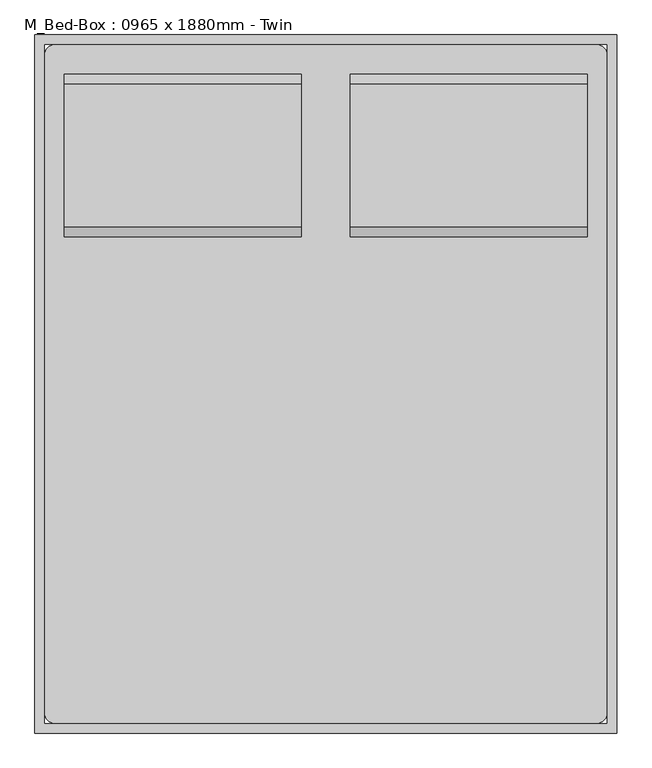
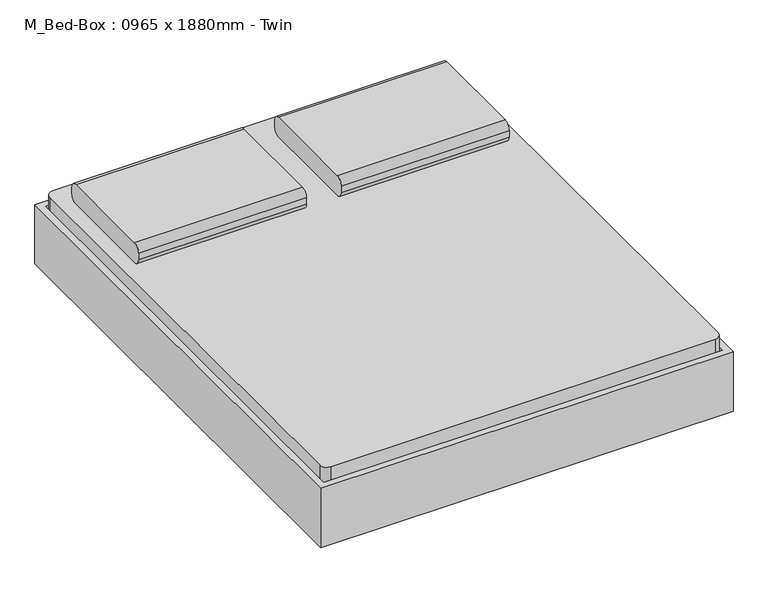
"""IFC4 building model written with IfcOpenShell, lengths in millimetres: furniture geometry, M_Bed-Box : 0965 x 1880mm - Twin."""

from ifc_helpers import new_model, si_unit, point, frame, frame_2d, origin, place, context, project, spatial, polyline, circle_curve, trimmed, segment, composite_curve, outline, extrude, source, transform, mapped, element, save
from ifc_brep_helpers import plane_surface, cylinder_surface, revolved_surface, advanced_brep


def m_bed_box_0965_x_1880mm_twin_f2e49195(model_context):
    return source(origin(), model_context, "Body", "SolidModel", [
        extrude(outline(composite_curve([segment(polyline([(538.5704918, 406.4), (170.2704918, 406.4)]), True, "CONTINUOUS"), segment(trimmed(circle_curve(frame_2d((170.2704918, 431.8)), 25.4), [point((170.2704918, 406.4))], [point((144.8704918, 431.8))], False, "CARTESIAN"), True, "CONTINUOUS"), segment(polyline([(144.8704918, 431.8), (144.8704918, 457.2)]), True, "CONTINUOUS"), segment(trimmed(circle_curve(frame_2d((170.2704918, 457.2)), 25.4), [point((144.8704918, 457.2))], [point((170.2704918, 482.6))], False, "CARTESIAN"), True, "CONTINUOUS"), segment(polyline([(170.2704918, 482.6), (538.5704918, 482.6)]), True, "CONTINUOUS"), segment(trimmed(circle_curve(frame_2d((538.5704918, 457.2)), 25.4), [point((538.5704918, 482.6))], [point((563.9704918, 457.2))], False, "CARTESIAN"), True, "CONTINUOUS"), segment(polyline([(563.9704918, 457.2), (563.9704918, 431.8)]), True, "CONTINUOUS"), segment(trimmed(circle_curve(frame_2d((538.5704918, 431.8)), 25.4), [point((563.9704918, 431.8))], [point((538.5704918, 406.4))], False, "CARTESIAN"), True, "CONTINUOUS")], self_intersect=False)), frame((402.652459, 0.0, 0.0), z_axis=(1.0, 0.0, 0.0), x_axis=(0.0, 1.0, 0.0)), (0.0, 0.0, 1.0), 610.3),
        extrude(outline(composite_curve([segment(polyline([(538.5704918, 406.4), (170.2704918, 406.4)]), True, "CONTINUOUS"), segment(trimmed(circle_curve(frame_2d((170.2704918, 431.8)), 25.4), [point((170.2704918, 406.4))], [point((144.8704918, 431.8))], False, "CARTESIAN"), True, "CONTINUOUS"), segment(polyline([(144.8704918, 431.8), (144.8704918, 457.2)]), True, "CONTINUOUS"), segment(trimmed(circle_curve(frame_2d((170.2704918, 457.2)), 25.4), [point((144.8704918, 457.2))], [point((170.2704918, 482.6))], False, "CARTESIAN"), True, "CONTINUOUS"), segment(polyline([(170.2704918, 482.6), (538.5704918, 482.6)]), True, "CONTINUOUS"), segment(trimmed(circle_curve(frame_2d((538.5704918, 457.2)), 25.4), [point((538.5704918, 482.6))], [point((563.9704918, 457.2))], False, "CARTESIAN"), True, "CONTINUOUS"), segment(polyline([(563.9704918, 457.2), (563.9704918, 431.8)]), True, "CONTINUOUS"), segment(trimmed(circle_curve(frame_2d((538.5704918, 431.8)), 25.4), [point((563.9704918, 431.8))], [point((538.5704918, 406.4))], False, "CARTESIAN"), True, "CONTINUOUS")], self_intersect=False)), frame((-334.647541, 0.0, 0.0), z_axis=(1.0, 0.0, 0.0), x_axis=(0.0, 1.0, 0.0)), (0.0, 0.0, 1.0), 610.3),
        advanced_brep(
        [(-385.1231784, 411.5704918, 177.8), (-385.1231784, 335.3704918, 177.8), (-385.1231784, 335.3704918, 196.85), (-385.1231784, 411.5704918, 196.85), (-334.3231784, 411.5704918, 177.8), (-334.3231784, 335.3704918, 177.8), (-322.1869899, 335.3704918, 196.85), (-322.1869899, 411.5704918, 196.85), (-258.2523099, 411.5704918, 14.6654962), (-258.2523099, 335.3704918, 14.6654962), (-240.9871466, 335.3704918, 22.716374), (-240.9871466, 411.5704918, 22.716374), (-235.2320921, 335.3704918, 0.0), (-235.2320921, 411.5704918, 0.0), (-235.2320921, 335.3704918, 19.05), (-235.2320921, 411.5704918, 19.05), (-156.6195862, 411.5704918, 0.0), (-156.6195862, 335.3704918, 0.0), (-156.6195862, 335.3704918, 19.05), (-156.6195862, 411.5704918, 19.05), (-143.9195862, 335.3704918, 3.4029547), (-143.9195862, 411.5704918, 3.4029547), (-153.4445862, 335.3704918, 19.9007387), (-153.4445862, 411.5704918, 19.9007387), (-83.822541, 411.5704918, 38.1), (-83.822541, 335.3704918, 38.1), (-88.9269731, 335.3704918, 57.15), (-88.9269731, 411.5704918, 57.15), (762.4518216, 411.5704918, 38.1), (762.4518216, 335.3704918, 38.1), (767.5562537, 335.3704918, 57.15), (767.5562537, 411.5704918, 57.15), (822.5488669, 411.5704918, 3.4029547), (822.5488669, 335.3704918, 3.4029547), (832.0738669, 335.3704918, 19.9007387), (832.0738669, 411.5704918, 19.9007387), (835.2488669, 335.3704918, 0.0), (835.2488669, 411.5704918, 0.0), (835.2488669, 335.3704918, 19.05), (835.2488669, 411.5704918, 19.05), (913.8613728, 411.5704918, 0.0), (913.8613728, 335.3704918, 0.0), (913.8613728, 335.3704918, 19.05), (913.8613728, 411.5704918, 19.05), (936.8815906, 335.3704918, 14.6654962), (936.8815906, 411.5704918, 14.6654962), (919.6164272, 335.3704918, 22.716374), (919.6164272, 411.5704918, 22.716374), (1012.952459, 411.5704918, 177.8), (1012.952459, 335.3704918, 177.8), (1000.8162705, 335.3704918, 196.85), (1000.8162705, 411.5704918, 196.85), (1063.752459, 411.5704918, 177.8), (1063.752459, 411.5704918, 196.85), (1063.752459, 335.3704918, 196.85), (1063.752459, 335.3704918, 177.8)],
        [
            (0, 1),
            (1, 2),
            (2, 3),
            (3, 0),
            (0, 4),
            (4, 5),
            (5, 1),
            (5, 6),
            (6, 2),
            (6, 7),
            (7, 3),
            (7, 4),
            (4, 8),
            (8, 9),
            (9, 5),
            (9, 10),
            (10, 6),
            (10, 11),
            (11, 7),
            (11, 8),
            (12, 9, circle_curve(frame((-235.2320921, 335.3704918, 25.4), z_axis=(0.0, 1.0, 0.0), x_axis=(-0.9063077870366488, 0.0, -0.4226182617407019)), 25.4)),
            (8, 13, circle_curve(frame((-235.2320921, 411.5704918, 25.4), z_axis=(0.0, -1.0, 0.0), x_axis=(-0.9063077870366488, 0.0, -0.4226182617407019)), 25.4)),
            (13, 12),
            (14, 10, circle_curve(frame((-235.2320921, 335.3704918, 25.4), z_axis=(0.0, 1.0, 0.0), x_axis=(-0.9063077870366488, 0.0, -0.4226182617407019)), 6.35)),
            (12, 14),
            (15, 11, circle_curve(frame((-235.2320921, 411.5704918, 25.4), z_axis=(0.0, 1.0, 0.0), x_axis=(-0.9063077870366488, 0.0, -0.4226182617407019)), 6.35)),
            (14, 15),
            (15, 13),
            (13, 16),
            (16, 17),
            (17, 12),
            (17, 18),
            (18, 14),
            (18, 19),
            (19, 15),
            (19, 16),
            (20, 17, circle_curve(frame((-156.6195862, 335.3704918, 25.4), z_axis=(0.0, 1.0, 0.0), x_axis=(0.0, 0.0, -1.0)), 25.4)),
            (16, 21, circle_curve(frame((-156.6195862, 411.5704918, 25.4), z_axis=(0.0, -1.0, 0.0), x_axis=(0.0, 0.0, -1.0)), 25.4)),
            (21, 20),
            (22, 18, circle_curve(frame((-156.6195862, 335.3704918, 25.4), z_axis=(0.0, 1.0, 0.0), x_axis=(0.0, 0.0, -1.0)), 6.35)),
            (20, 22),
            (23, 19, circle_curve(frame((-156.6195862, 411.5704918, 25.4), z_axis=(0.0, 1.0, 0.0), x_axis=(0.0, 0.0, -1.0)), 6.35)),
            (22, 23),
            (23, 21),
            (21, 24),
            (24, 25),
            (25, 20),
            (25, 26),
            (26, 22),
            (26, 27),
            (27, 23),
            (27, 24),
            (24, 28),
            (28, 29),
            (29, 25),
            (29, 30),
            (30, 26),
            (30, 31),
            (31, 27),
            (31, 28),
            (28, 32),
            (32, 33),
            (33, 29),
            (33, 34),
            (34, 30),
            (34, 35),
            (35, 31),
            (35, 32),
            (36, 33, circle_curve(frame((835.2488669, 335.3704918, 25.4), z_axis=(0.0, 1.0, 0.0), x_axis=(-0.5000000000000463, 0.0, -0.8660254037844118)), 25.4)),
            (32, 37, circle_curve(frame((835.2488669, 411.5704918, 25.4), z_axis=(0.0, -1.0, 0.0), x_axis=(-0.5000000000000463, 0.0, -0.8660254037844118)), 25.4)),
            (37, 36),
            (38, 34, circle_curve(frame((835.2488669, 335.3704918, 25.4), z_axis=(0.0, 1.0, 0.0), x_axis=(-0.5000000000000463, 0.0, -0.8660254037844118)), 6.35)),
            (36, 38),
            (39, 35, circle_curve(frame((835.2488669, 411.5704918, 25.4), z_axis=(0.0, 1.0, 0.0), x_axis=(-0.5000000000000463, 0.0, -0.8660254037844118)), 6.35)),
            (38, 39),
            (39, 37),
            (37, 40),
            (40, 41),
            (41, 36),
            (41, 42),
            (42, 38),
            (42, 43),
            (43, 39),
            (43, 40),
            (44, 41, circle_curve(frame((913.8613728, 335.3704918, 25.4), z_axis=(0.0, 1.0, 0.0), x_axis=(0.0, 0.0, -1.0)), 25.4)),
            (40, 45, circle_curve(frame((913.8613728, 411.5704918, 25.4), z_axis=(0.0, -1.0, 0.0), x_axis=(0.0, 0.0, -1.0)), 25.4)),
            (45, 44),
            (46, 42, circle_curve(frame((913.8613728, 335.3704918, 25.4), z_axis=(0.0, 1.0, 0.0), x_axis=(0.0, 0.0, -1.0)), 6.35)),
            (44, 46),
            (47, 43, circle_curve(frame((913.8613728, 411.5704918, 25.4), z_axis=(0.0, 1.0, 0.0), x_axis=(0.0, 0.0, -1.0)), 6.35)),
            (46, 47),
            (47, 45),
            (45, 48),
            (48, 49),
            (49, 44),
            (49, 50),
            (50, 46),
            (50, 51),
            (51, 47),
            (51, 48),
            (52, 53),
            (53, 54),
            (54, 55),
            (55, 52),
            (48, 52),
            (55, 49),
            (54, 50),
            (53, 51),
        ],
        [
            plane_surface(frame((-385.1231784, 665.5704918, -152.9490627), z_axis=(-1.0, 0.0, 0.0), x_axis=(0.0, 1.0, 0.0))),
            plane_surface(frame((-385.1231784, 411.5704918, 177.8), z_axis=(0.0, 0.0, -1.0), x_axis=(1.0, 0.0, 0.0))),
            plane_surface(frame((-385.1231784, 335.3704918, 177.8), z_axis=(0.0, -1.0, 0.0), x_axis=(1.0, 0.0, 0.0))),
            plane_surface(frame((-385.1231784, 335.3704918, 196.85), z_axis=(0.0, 0.0, 1.0), x_axis=(1.0, 0.0, 0.0))),
            plane_surface(frame((-385.1231784, 411.5704918, 196.85), z_axis=(0.0, 1.0, 0.0), x_axis=(1.0, 0.0, 0.0))),
            plane_surface(frame((-334.3231784, 411.5704918, 177.8), z_axis=(-0.9063077870366485, 0.0, -0.4226182617407027), x_axis=(0.4226182617407027, 0.0, -0.9063077870366485))),
            plane_surface(frame((-334.3231784, 335.3704918, 177.8), z_axis=(0.0, -1.0, 0.0), x_axis=(0.4226182617407027, 0.0, -0.9063077870366485))),
            plane_surface(frame((-322.1869899, 335.3704918, 196.85), z_axis=(0.9063077870366486, 0.0, 0.4226182617407026), x_axis=(0.4226182617407026, 0.0, -0.9063077870366486))),
            plane_surface(frame((-322.1869899, 411.5704918, 196.85), z_axis=(0.0, 1.0, 0.0), x_axis=(0.4226182617407027, 0.0, -0.9063077870366485))),
            cylinder_surface(frame((-235.2320921, 665.5704918, 25.4), z_axis=(0.0, -1.0, 0.0), x_axis=(-0.9063077870366488, 0.0, -0.4226182617407019)), 25.4),
            plane_surface(frame((-235.2320921, 335.3704918, 25.4), z_axis=(0.0, -1.0, 0.0), x_axis=(-0.9063077870366488, 0.0, -0.4226182617407019))),
            revolved_surface(polyline([(-240.9871465476827, 335.3704918, 22.716374037946544), (-240.9871465476827, 411.5704918, 22.716374037946544)]), (-235.2320921, 665.5704918, 25.4), (0.0, -1.0, 0.0)),
            plane_surface(frame((-235.2320921, 411.5704918, 25.4), z_axis=(0.0, 1.0, 0.0), x_axis=(-0.9063077870366488, 0.0, -0.4226182617407019))),
            plane_surface(frame((-235.2320921, 411.5704918, 0.0), z_axis=(0.0, 0.0, -1.0), x_axis=(1.0, 0.0, 0.0))),
            plane_surface(frame((-235.2320921, 335.3704918, 0.0), z_axis=(0.0, -1.0, 0.0), x_axis=(1.0, 0.0, 0.0))),
            plane_surface(frame((-235.2320921, 335.3704918, 19.05), z_axis=(0.0, 0.0, 1.0), x_axis=(1.0, 0.0, 0.0))),
            plane_surface(frame((-235.2320921, 411.5704918, 19.05), z_axis=(0.0, 1.0, 0.0), x_axis=(1.0, 0.0, 0.0))),
            cylinder_surface(frame((-156.6195862, 665.5704918, 25.4), z_axis=(0.0, -1.0, 0.0), x_axis=(0.0, 0.0, -1.0)), 25.4),
            plane_surface(frame((-156.6195862, 335.3704918, 25.4), z_axis=(0.0, -1.0, 0.0), x_axis=(0.0, 0.0, -1.0))),
            revolved_surface(polyline([(-156.6195862, 335.3704918, 19.049999999999997), (-156.6195862, 411.5704918, 19.049999999999997)]), (-156.6195862, 665.5704918, 25.4), (0.0, -1.0, 0.0)),
            plane_surface(frame((-156.6195862, 411.5704918, 25.4), z_axis=(0.0, 1.0, 0.0), x_axis=(0.0, 0.0, -1.0))),
            plane_surface(frame((-143.9195862, 411.5704918, 3.4029547), z_axis=(0.4999999999998775, 0.0, -0.8660254037845093), x_axis=(0.8660254037845093, 0.0, 0.4999999999998775))),
            plane_surface(frame((-143.9195862, 335.3704918, 3.4029547), z_axis=(0.0, -1.0, 0.0), x_axis=(0.8660254037845092, 0.0, 0.49999999999987776))),
            plane_surface(frame((-153.4445862, 335.3704918, 19.9007387), z_axis=(-0.4999999999998776, 0.0, 0.8660254037845093), x_axis=(0.8660254037845093, 0.0, 0.4999999999998776))),
            plane_surface(frame((-153.4445862, 411.5704918, 19.9007387), z_axis=(0.0, 1.0, 0.0), x_axis=(0.8660254037845095, 0.0, 0.4999999999998772))),
            plane_surface(frame((-83.822541, 411.5704918, 38.1), z_axis=(0.0, 0.0, -1.0), x_axis=(1.0, 0.0, 0.0))),
            plane_surface(frame((-83.822541, 335.3704918, 38.1), z_axis=(0.0, -1.0, 0.0), x_axis=(1.0, 0.0, 0.0))),
            plane_surface(frame((-88.9269731, 335.3704918, 57.15), z_axis=(0.0, 0.0, 1.0), x_axis=(1.0, 0.0, 0.0))),
            plane_surface(frame((-88.9269731, 411.5704918, 57.15), z_axis=(0.0, 1.0, 0.0), x_axis=(1.0, 0.0, 0.0))),
            plane_surface(frame((762.4518216, 411.5704918, 38.1), z_axis=(-0.5000000000000455, 0.0, -0.8660254037844124), x_axis=(0.8660254037844124, 0.0, -0.5000000000000455))),
            plane_surface(frame((762.4518216, 335.3704918, 38.1), z_axis=(0.0, -1.0000000000000002, 0.0), x_axis=(0.8660254037844132, 0.0, -0.5000000000000443))),
            plane_surface(frame((767.5562537, 335.3704918, 57.15), z_axis=(0.500000000000045, 0.0, 0.8660254037844127), x_axis=(0.8660254037844127, 0.0, -0.500000000000045))),
            plane_surface(frame((767.5562537, 411.5704918, 57.15), z_axis=(0.0, 1.0000000000000002, 0.0), x_axis=(0.8660254037844123, 0.0, -0.5000000000000459))),
            cylinder_surface(frame((835.2488669, 665.5704918, 25.4), z_axis=(0.0, -1.0, 0.0), x_axis=(-0.5000000000000463, 0.0, -0.8660254037844118)), 25.4),
            plane_surface(frame((835.2488669, 335.3704918, 25.4), z_axis=(0.0, -1.0000000000000002, 0.0), x_axis=(-0.5000000000000464, 0.0, -0.866025403784412))),
            revolved_surface(polyline([(832.0738668999998, 335.3704918, 19.90073868596898), (832.0738668999998, 411.5704918, 19.90073868596898)]), (835.2488669, 665.5704918, 25.4), (0.0, -1.0, 0.0)),
            plane_surface(frame((835.2488669, 411.5704918, 25.4), z_axis=(0.0, 1.0000000000000002, 0.0), x_axis=(-0.5000000000000464, 0.0, -0.866025403784412))),
            plane_surface(frame((835.2488669, 411.5704918, 0.0), z_axis=(0.0, 0.0, -1.0), x_axis=(1.0, 0.0, 0.0))),
            plane_surface(frame((835.2488669, 335.3704918, 0.0), z_axis=(0.0, -1.0, 0.0), x_axis=(1.0, 0.0, 0.0))),
            plane_surface(frame((835.2488669, 335.3704918, 19.05), z_axis=(0.0, 0.0, 1.0), x_axis=(1.0, 0.0, 0.0))),
            plane_surface(frame((835.2488669, 411.5704918, 19.05), z_axis=(0.0, 1.0, 0.0), x_axis=(1.0, 0.0, 0.0))),
            cylinder_surface(frame((913.8613728, 665.5704918, 25.4), z_axis=(0.0, -1.0, 0.0), x_axis=(0.0, 0.0, -1.0)), 25.4),
            plane_surface(frame((913.8613728, 335.3704918, 25.4), z_axis=(0.0, -1.0, 0.0), x_axis=(0.0, 0.0, -1.0))),
            revolved_surface(polyline([(913.8613728, 335.3704918, 19.049999999999997), (913.8613728, 411.5704918, 19.049999999999997)]), (913.8613728, 665.5704918, 25.4), (0.0, -1.0, 0.0)),
            plane_surface(frame((913.8613728, 411.5704918, 25.4), z_axis=(0.0, 1.0, 0.0), x_axis=(0.0, 0.0, -1.0))),
            plane_surface(frame((936.8815906, 411.5704918, 14.6654962), z_axis=(0.9063077870366809, 0.0, -0.42261826174063305), x_axis=(0.42261826174063305, 0.0, 0.9063077870366809))),
            plane_surface(frame((936.8815906, 335.3704918, 14.6654962), z_axis=(0.0, -1.0, 0.0), x_axis=(0.4226182617406331, 0.0, 0.9063077870366809))),
            plane_surface(frame((919.6164272, 335.3704918, 22.716374), z_axis=(-0.9063077870366807, 0.0, 0.4226182617406336), x_axis=(0.4226182617406336, 0.0, 0.9063077870366807))),
            plane_surface(frame((919.6164272, 411.5704918, 22.716374), z_axis=(0.0, 1.0000000000000002, 0.0), x_axis=(0.422618261740634, 0.0, 0.9063077870366806))),
            plane_surface(frame((1063.752459, 665.5704918, -152.9490627), z_axis=(1.0, 0.0, 0.0), x_axis=(0.0, 1.0, 0.0))),
            plane_surface(frame((1012.952459, 411.5704918, 177.8), z_axis=(0.0, 0.0, -1.0), x_axis=(1.0, 0.0, 0.0))),
            plane_surface(frame((1012.952459, 335.3704918, 177.8), z_axis=(0.0, -1.0, 0.0), x_axis=(1.0, 0.0, 0.0))),
            plane_surface(frame((1000.8162705, 335.3704918, 196.85), z_axis=(0.0, 0.0, 1.0), x_axis=(1.0, 0.0, 0.0))),
            plane_surface(frame((1000.8162705, 411.5704918, 196.85), z_axis=(0.0, 1.0, 0.0), x_axis=(1.0, 0.0, 0.0))),
        ],
        [
            (0, [[1, 2, 3, 4]]),
            (1, [[-1, 5, 6, 7]]),
            (2, [[-2, -7, 8, 9]]),
            (3, [[-3, -9, 10, 11]]),
            (4, [[-4, -11, 12, -5]]),
            (5, [[-6, 13, 14, 15]]),
            (6, [[-8, -15, 16, 17]]),
            (7, [[-10, -17, 18, 19]]),
            (8, [[-12, -19, 20, -13]]),
            (9, [[21, -14, 22, 23]]),
            (10, [[24, -16, -21, 25]]),
            (11, [[26, -18, -24, 27]]),
            (12, [[-22, -20, -26, 28]]),
            (13, [[-23, 29, 30, 31]]),
            (14, [[-25, -31, 32, 33]]),
            (15, [[-27, -33, 34, 35]]),
            (16, [[-28, -35, 36, -29]]),
            (17, [[37, -30, 38, 39]]),
            (18, [[40, -32, -37, 41]]),
            (19, [[42, -34, -40, 43]]),
            (20, [[-38, -36, -42, 44]]),
            (21, [[-39, 45, 46, 47]]),
            (22, [[-41, -47, 48, 49]]),
            (23, [[-43, -49, 50, 51]]),
            (24, [[-44, -51, 52, -45]]),
            (25, [[-46, 53, 54, 55]]),
            (26, [[-48, -55, 56, 57]]),
            (27, [[-50, -57, 58, 59]]),
            (28, [[-52, -59, 60, -53]]),
            (29, [[-54, 61, 62, 63]]),
            (30, [[-56, -63, 64, 65]]),
            (31, [[-58, -65, 66, 67]]),
            (32, [[-60, -67, 68, -61]]),
            (33, [[69, -62, 70, 71]]),
            (34, [[72, -64, -69, 73]]),
            (35, [[74, -66, -72, 75]]),
            (36, [[-70, -68, -74, 76]]),
            (37, [[-71, 77, 78, 79]]),
            (38, [[-73, -79, 80, 81]]),
            (39, [[-75, -81, 82, 83]]),
            (40, [[-76, -83, 84, -77]]),
            (41, [[85, -78, 86, 87]]),
            (42, [[88, -80, -85, 89]]),
            (43, [[90, -82, -88, 91]]),
            (44, [[-86, -84, -90, 92]]),
            (45, [[-87, 93, 94, 95]]),
            (46, [[-89, -95, 96, 97]]),
            (47, [[-91, -97, 98, 99]]),
            (48, [[-92, -99, 100, -93]]),
            (49, [[101, 102, 103, 104]]),
            (50, [[-94, 105, -104, 106]]),
            (51, [[-96, -106, -103, 107]]),
            (52, [[-98, -107, -102, 108]]),
            (53, [[-100, -108, -101, -105]]),
        ],
    ),
        extrude(outline(composite_curve([segment(polyline([(-360.047541, 640.1704918), (1038.352459, 640.1704918)]), True, "CONTINUOUS"), segment(trimmed(circle_curve(frame_2d((1038.352459, 614.7704918)), 25.4), [point((1038.352459, 640.1704918))], [point((1063.752459, 614.7704918))], False, "CARTESIAN"), True, "CONTINUOUS"), segment(polyline([(1063.752459, 614.7704918), (1063.752459, -1083.6295082)]), True, "CONTINUOUS"), segment(trimmed(circle_curve(frame_2d((1038.352459, -1083.6295082)), 25.4), [point((1063.752459, -1083.6295082))], [point((1038.352459, -1109.0295082))], False, "CARTESIAN"), True, "CONTINUOUS"), segment(polyline([(1038.352459, -1109.0295082), (-360.047541, -1109.0295082)]), True, "CONTINUOUS"), segment(trimmed(circle_curve(frame_2d((-360.047541, -1083.6295082)), 25.4), [point((-360.047541, -1109.0295082))], [point((-385.447541, -1083.6295082))], False, "CARTESIAN"), True, "CONTINUOUS"), segment(polyline([(-385.447541, -1083.6295082), (-385.447541, 614.7704918)]), True, "CONTINUOUS"), segment(trimmed(circle_curve(frame_2d((-360.047541, 614.7704918)), 25.4), [point((-385.447541, 614.7704918))], [point((-360.047541, 640.1704918))], False, "CARTESIAN"), True, "CONTINUOUS")], self_intersect=False)), frame((0.0, 0.0, 203.2), z_axis=(0.0, 0.0, 1.0), x_axis=(1.0, 0.0, 0.0)), (0.0, 0.0, 1.0), 203.2),
        advanced_brep(
        [(-385.447541, -829.6295082, 196.85), (-385.447541, -829.6295082, 177.8), (-385.447541, -905.8295082, 177.8), (-385.447541, -905.8295082, 196.85), (-322.5113525, -829.6295082, 196.85), (-334.647541, -829.6295082, 177.8), (-334.647541, -905.8295082, 177.8), (-322.5113525, -905.8295082, 196.85), (-241.3115092, -829.6295082, 22.716374), (-258.5766725, -829.6295082, 14.6654962), (-258.5766725, -905.8295082, 14.6654962), (-241.3115092, -905.8295082, 22.716374), (-235.5564547, -829.6295082, 0.0), (-235.5564547, -829.6295082, 19.05), (-235.5564547, -905.8295082, 0.0), (-235.5564547, -905.8295082, 19.05), (-156.9439489, -829.6295082, 19.05), (-156.9439489, -829.6295082, 0.0), (-156.9439489, -905.8295082, 0.0), (-156.9439489, -905.8295082, 19.05), (-144.2439489, -829.6295082, 3.4029547), (-153.7689489, -829.6295082, 19.9007387), (-144.2439489, -905.8295082, 3.4029547), (-153.7689489, -905.8295082, 19.9007387), (-89.2513357, -829.6295082, 57.15), (-84.1469036, -829.6295082, 38.1), (-84.1469036, -905.8295082, 38.1), (-89.2513357, -905.8295082, 57.15), (767.5562537, -829.6295082, 57.15), (762.4518216, -829.6295082, 38.1), (762.4518216, -905.8295082, 38.1), (767.5562537, -905.8295082, 57.15), (832.0738669, -829.6295082, 19.9007387), (822.5488669, -829.6295082, 3.4029547), (822.5488669, -905.8295082, 3.4029547), (832.0738669, -905.8295082, 19.9007387), (835.2488669, -829.6295082, 0.0), (835.2488669, -829.6295082, 19.05), (835.2488669, -905.8295082, 0.0), (835.2488669, -905.8295082, 19.05), (913.8613728, -829.6295082, 19.05), (913.8613728, -829.6295082, 0.0), (913.8613728, -905.8295082, 0.0), (913.8613728, -905.8295082, 19.05), (936.8815906, -829.6295082, 14.6654962), (919.6164272, -829.6295082, 22.716374), (936.8815906, -905.8295082, 14.6654962), (919.6164272, -905.8295082, 22.716374), (1000.8162705, -829.6295082, 196.85), (1012.952459, -829.6295082, 177.8), (1012.952459, -905.8295082, 177.8), (1000.8162705, -905.8295082, 196.85), (1063.752459, -829.6295082, 196.85), (1063.752459, -905.8295082, 196.85), (1063.752459, -905.8295082, 177.8), (1063.752459, -829.6295082, 177.8)],
        [
            (0, 1),
            (1, 2),
            (2, 3),
            (3, 0),
            (0, 4),
            (4, 5),
            (5, 1),
            (5, 6),
            (6, 2),
            (6, 7),
            (7, 3),
            (7, 4),
            (4, 8),
            (8, 9),
            (9, 5),
            (9, 10),
            (10, 6),
            (10, 11),
            (11, 7),
            (11, 8),
            (12, 9, circle_curve(frame((-235.5564547, -829.6295082, 25.4), z_axis=(0.0, 1.0, 0.0), x_axis=(-0.906307787036664, 0.0, -0.4226182617406693)), 25.4)),
            (8, 13, circle_curve(frame((-235.5564547, -829.6295082, 25.4), z_axis=(0.0, -1.0, 0.0), x_axis=(-0.906307787036664, 0.0, -0.4226182617406693)), 6.35)),
            (13, 12),
            (14, 10, circle_curve(frame((-235.5564547, -905.8295082, 25.4), z_axis=(0.0, 1.0, 0.0), x_axis=(-0.906307787036664, 0.0, -0.4226182617406693)), 25.4)),
            (12, 14),
            (15, 11, circle_curve(frame((-235.5564547, -905.8295082, 25.4), z_axis=(0.0, 1.0, 0.0), x_axis=(-0.906307787036664, 0.0, -0.4226182617406693)), 6.35)),
            (14, 15),
            (15, 13),
            (13, 16),
            (16, 17),
            (17, 12),
            (17, 18),
            (18, 14),
            (18, 19),
            (19, 15),
            (19, 16),
            (20, 17, circle_curve(frame((-156.9439489, -829.6295082, 25.4), z_axis=(0.0, 1.0, 0.0), x_axis=(0.0, 0.0, -1.0)), 25.4)),
            (16, 21, circle_curve(frame((-156.9439489, -829.6295082, 25.4), z_axis=(0.0, -1.0, 0.0), x_axis=(0.0, 0.0, -1.0)), 6.35)),
            (21, 20),
            (22, 18, circle_curve(frame((-156.9439489, -905.8295082, 25.4), z_axis=(0.0, 1.0, 0.0), x_axis=(0.0, 0.0, -1.0)), 25.4)),
            (20, 22),
            (23, 19, circle_curve(frame((-156.9439489, -905.8295082, 25.4), z_axis=(0.0, 1.0, 0.0), x_axis=(0.0, 0.0, -1.0)), 6.35)),
            (22, 23),
            (23, 21),
            (21, 24),
            (24, 25),
            (25, 20),
            (25, 26),
            (26, 22),
            (26, 27),
            (27, 23),
            (27, 24),
            (24, 28),
            (28, 29),
            (29, 25),
            (29, 30),
            (30, 26),
            (30, 31),
            (31, 27),
            (31, 28),
            (28, 32),
            (32, 33),
            (33, 29),
            (33, 34),
            (34, 30),
            (34, 35),
            (35, 31),
            (35, 32),
            (36, 33, circle_curve(frame((835.2488669, -829.6295082, 25.4), z_axis=(0.0, 1.0, 0.0), x_axis=(-0.5000000000000525, 0.0, -0.8660254037844083)), 25.4)),
            (32, 37, circle_curve(frame((835.2488669, -829.6295082, 25.4), z_axis=(0.0, -1.0, 0.0), x_axis=(-0.5000000000000525, 0.0, -0.8660254037844083)), 6.35)),
            (37, 36),
            (38, 34, circle_curve(frame((835.2488669, -905.8295082, 25.4), z_axis=(0.0, 1.0, 0.0), x_axis=(-0.5000000000000525, 0.0, -0.8660254037844083)), 25.4)),
            (36, 38),
            (39, 35, circle_curve(frame((835.2488669, -905.8295082, 25.4), z_axis=(0.0, 1.0, 0.0), x_axis=(-0.5000000000000525, 0.0, -0.8660254037844083)), 6.35)),
            (38, 39),
            (39, 37),
            (37, 40),
            (40, 41),
            (41, 36),
            (41, 42),
            (42, 38),
            (42, 43),
            (43, 39),
            (43, 40),
            (44, 41, circle_curve(frame((913.8613728, -829.6295082, 25.4), z_axis=(0.0, 1.0, 0.0), x_axis=(0.0, 0.0, -1.0)), 25.4)),
            (40, 45, circle_curve(frame((913.8613728, -829.6295082, 25.4), z_axis=(0.0, -1.0, 0.0), x_axis=(0.0, 0.0, -1.0)), 6.35)),
            (45, 44),
            (46, 42, circle_curve(frame((913.8613728, -905.8295082, 25.4), z_axis=(0.0, 1.0, 0.0), x_axis=(0.0, 0.0, -1.0)), 25.4)),
            (44, 46),
            (47, 43, circle_curve(frame((913.8613728, -905.8295082, 25.4), z_axis=(0.0, 1.0, 0.0), x_axis=(0.0, 0.0, -1.0)), 6.35)),
            (46, 47),
            (47, 45),
            (45, 48),
            (48, 49),
            (49, 44),
            (49, 50),
            (50, 46),
            (50, 51),
            (51, 47),
            (51, 48),
            (52, 53),
            (53, 54),
            (54, 55),
            (55, 52),
            (48, 52),
            (55, 49),
            (54, 50),
            (53, 51),
        ],
        [
            plane_surface(frame((-385.447541, -1134.4295082, -127.5947323), z_axis=(-1.0, 0.0, 0.0), x_axis=(0.0, 1.0, 0.0))),
            plane_surface(frame((-385.447541, -829.6295082, 196.85), z_axis=(0.0, 1.0, 0.0), x_axis=(1.0, 0.0, 0.0))),
            plane_surface(frame((-385.447541, -829.6295082, 177.8), z_axis=(0.0, 0.0, -1.0), x_axis=(1.0, 0.0, 0.0))),
            plane_surface(frame((-385.447541, -905.8295082, 177.8), z_axis=(0.0, -1.0, 0.0), x_axis=(1.0, 0.0, 0.0))),
            plane_surface(frame((-385.447541, -905.8295082, 196.85), z_axis=(0.0, 0.0, 1.0), x_axis=(1.0, 0.0, 0.0))),
            plane_surface(frame((-322.5113525, -829.6295082, 196.85), z_axis=(0.0, 1.0000000000000002, 0.0), x_axis=(0.42261826174067135, 0.0, -0.9063077870366631))),
            plane_surface(frame((-334.647541, -829.6295082, 177.8), z_axis=(-0.906307787036663, 0.0, -0.42261826174067146), x_axis=(0.42261826174067146, 0.0, -0.906307787036663))),
            plane_surface(frame((-334.647541, -905.8295082, 177.8), z_axis=(0.0, -1.0, 0.0), x_axis=(0.42261826174067174, 0.0, -0.9063077870366629))),
            plane_surface(frame((-322.5113525, -905.8295082, 196.85), z_axis=(0.906307787036663, 0.0, 0.4226182617406716), x_axis=(0.4226182617406716, 0.0, -0.906307787036663))),
            plane_surface(frame((-235.5564547, -829.6295082, 25.4), z_axis=(0.0, 1.0, 0.0), x_axis=(-0.906307787036664, 0.0, -0.4226182617406693))),
            cylinder_surface(frame((-235.5564547, -1134.4295082, 25.4), z_axis=(0.0, -1.0, 0.0), x_axis=(-0.906307787036664, 0.0, -0.4226182617406693)), 25.4),
            plane_surface(frame((-235.5564547, -905.8295082, 25.4), z_axis=(0.0, -1.0, 0.0), x_axis=(-0.906307787036664, 0.0, -0.4226182617406693))),
            revolved_surface(polyline([(-241.3115091476828, -905.8295082, 22.71637403794675), (-241.3115091476828, -829.6295082, 22.71637403794675)]), (-235.5564547, -1134.4295082, 25.4), (0.0, -1.0, 0.0)),
            plane_surface(frame((-235.5564547, -829.6295082, 19.05), z_axis=(0.0, 1.0, 0.0), x_axis=(1.0, 0.0, 0.0))),
            plane_surface(frame((-235.5564547, -829.6295082, 0.0), z_axis=(0.0, 0.0, -1.0), x_axis=(1.0, 0.0, 0.0))),
            plane_surface(frame((-235.5564547, -905.8295082, 0.0), z_axis=(0.0, -1.0, 0.0), x_axis=(1.0, 0.0, 0.0))),
            plane_surface(frame((-235.5564547, -905.8295082, 19.05), z_axis=(0.0, 0.0, 1.0), x_axis=(1.0, 0.0, 0.0))),
            plane_surface(frame((-156.9439489, -829.6295082, 25.4), z_axis=(0.0, 1.0, 0.0), x_axis=(0.0, 0.0, -1.0))),
            cylinder_surface(frame((-156.9439489, -1134.4295082, 25.4), z_axis=(0.0, -1.0, 0.0), x_axis=(0.0, 0.0, -1.0)), 25.4),
            plane_surface(frame((-156.9439489, -905.8295082, 25.4), z_axis=(0.0, -1.0, 0.0), x_axis=(0.0, 0.0, -1.0))),
            revolved_surface(polyline([(-156.9439489, -905.8295082, 19.049999999999997), (-156.9439489, -829.6295082, 19.049999999999997)]), (-156.9439489, -1134.4295082, 25.4), (0.0, -1.0, 0.0)),
            plane_surface(frame((-153.7689489, -829.6295082, 19.9007387), z_axis=(0.0, 1.0, 0.0), x_axis=(0.8660254037844785, 0.0, 0.49999999999993117))),
            plane_surface(frame((-144.2439489, -829.6295082, 3.4029547), z_axis=(0.49999999999993167, 0.0, -0.8660254037844781), x_axis=(0.8660254037844781, 0.0, 0.49999999999993167))),
            plane_surface(frame((-144.2439489, -905.8295082, 3.4029547), z_axis=(0.0, -1.0000000000000002, 0.0), x_axis=(0.8660254037844782, 0.0, 0.49999999999993155))),
            plane_surface(frame((-153.7689489, -905.8295082, 19.9007387), z_axis=(-0.4999999999999309, 0.0, 0.8660254037844786), x_axis=(0.8660254037844786, 0.0, 0.4999999999999309))),
            plane_surface(frame((-89.2513357, -829.6295082, 57.15), z_axis=(0.0, 1.0, 0.0), x_axis=(1.0, 0.0, 0.0))),
            plane_surface(frame((-84.1469036, -829.6295082, 38.1), z_axis=(0.0, 0.0, -1.0), x_axis=(1.0, 0.0, 0.0))),
            plane_surface(frame((-84.1469036, -905.8295082, 38.1), z_axis=(0.0, -1.0, 0.0), x_axis=(1.0, 0.0, 0.0))),
            plane_surface(frame((-89.2513357, -905.8295082, 57.15), z_axis=(0.0, 0.0, 1.0), x_axis=(1.0, 0.0, 0.0))),
            plane_surface(frame((767.5562537, -829.6295082, 57.15), z_axis=(0.0, 1.0, 0.0), x_axis=(0.866025403784409, 0.0, -0.5000000000000515))),
            plane_surface(frame((762.4518216, -829.6295082, 38.1), z_axis=(-0.5000000000000513, 0.0, -0.8660254037844091), x_axis=(0.8660254037844091, 0.0, -0.5000000000000513))),
            plane_surface(frame((762.4518216, -905.8295082, 38.1), z_axis=(0.0, -1.0000000000000002, 0.0), x_axis=(0.8660254037844084, 0.0, -0.5000000000000526))),
            plane_surface(frame((767.5562537, -905.8295082, 57.15), z_axis=(0.5000000000000507, 0.0, 0.8660254037844094), x_axis=(0.8660254037844094, 0.0, -0.5000000000000507))),
            plane_surface(frame((835.2488669, -829.6295082, 25.4), z_axis=(0.0, 1.0000000000000002, 0.0), x_axis=(-0.5000000000000526, 0.0, -0.8660254037844084))),
            cylinder_surface(frame((835.2488669, -1134.4295082, 25.4), z_axis=(0.0, -1.0, 0.0), x_axis=(-0.5000000000000525, 0.0, -0.8660254037844083)), 25.4),
            plane_surface(frame((835.2488669, -905.8295082, 25.4), z_axis=(0.0, -1.0000000000000002, 0.0), x_axis=(-0.5000000000000526, 0.0, -0.8660254037844084))),
            revolved_surface(polyline([(832.0738668999998, -905.8295082, 19.900738685969007), (832.0738668999998, -829.6295082, 19.900738685969007)]), (835.2488669, -1134.4295082, 25.4), (0.0, -1.0, 0.0)),
            plane_surface(frame((835.2488669, -829.6295082, 19.05), z_axis=(0.0, 1.0, 0.0), x_axis=(1.0, 0.0, 0.0))),
            plane_surface(frame((835.2488669, -829.6295082, 0.0), z_axis=(0.0, 0.0, -1.0), x_axis=(1.0, 0.0, 0.0))),
            plane_surface(frame((835.2488669, -905.8295082, 0.0), z_axis=(0.0, -1.0, 0.0), x_axis=(1.0, 0.0, 0.0))),
            plane_surface(frame((835.2488669, -905.8295082, 19.05), z_axis=(0.0, 0.0, 1.0), x_axis=(1.0, 0.0, 0.0))),
            plane_surface(frame((913.8613728, -829.6295082, 25.4), z_axis=(0.0, 1.0, 0.0), x_axis=(0.0, 0.0, -1.0))),
            cylinder_surface(frame((913.8613728, -1134.4295082, 25.4), z_axis=(0.0, -1.0, 0.0), x_axis=(0.0, 0.0, -1.0)), 25.4),
            plane_surface(frame((913.8613728, -905.8295082, 25.4), z_axis=(0.0, -1.0, 0.0), x_axis=(0.0, 0.0, -1.0))),
            revolved_surface(polyline([(913.8613728, -905.8295082, 19.049999999999997), (913.8613728, -829.6295082, 19.049999999999997)]), (913.8613728, -1134.4295082, 25.4), (0.0, -1.0, 0.0)),
            plane_surface(frame((919.6164272, -829.6295082, 22.716374), z_axis=(0.0, 1.0, 0.0), x_axis=(0.4226182617405401, 0.0, 0.9063077870367242))),
            plane_surface(frame((936.8815906, -829.6295082, 14.6654962), z_axis=(0.9063077870367245, 0.0, -0.4226182617405395), x_axis=(0.4226182617405395, 0.0, 0.9063077870367245))),
            plane_surface(frame((936.8815906, -905.8295082, 14.6654962), z_axis=(0.0, -1.0, 0.0), x_axis=(0.4226182617405402, 0.0, 0.9063077870367242))),
            plane_surface(frame((919.6164272, -905.8295082, 22.716374), z_axis=(-0.9063077870367241, 0.0, 0.42261826174054035), x_axis=(0.42261826174054035, 0.0, 0.9063077870367241))),
            plane_surface(frame((1063.752459, -1134.4295082, -127.5947323), z_axis=(1.0, 0.0, 0.0), x_axis=(0.0, 1.0, 0.0))),
            plane_surface(frame((1000.8162705, -829.6295082, 196.85), z_axis=(0.0, 1.0, 0.0), x_axis=(1.0, 0.0, 0.0))),
            plane_surface(frame((1012.952459, -829.6295082, 177.8), z_axis=(0.0, 0.0, -1.0), x_axis=(1.0, 0.0, 0.0))),
            plane_surface(frame((1012.952459, -905.8295082, 177.8), z_axis=(0.0, -1.0, 0.0), x_axis=(1.0, 0.0, 0.0))),
            plane_surface(frame((1000.8162705, -905.8295082, 196.85), z_axis=(0.0, 0.0, 1.0), x_axis=(1.0, 0.0, 0.0))),
        ],
        [
            (0, [[1, 2, 3, 4]]),
            (1, [[-1, 5, 6, 7]]),
            (2, [[-2, -7, 8, 9]]),
            (3, [[-3, -9, 10, 11]]),
            (4, [[-4, -11, 12, -5]]),
            (5, [[-6, 13, 14, 15]]),
            (6, [[-8, -15, 16, 17]]),
            (7, [[-10, -17, 18, 19]]),
            (8, [[-12, -19, 20, -13]]),
            (9, [[21, -14, 22, 23]]),
            (10, [[24, -16, -21, 25]]),
            (11, [[26, -18, -24, 27]]),
            (12, [[-22, -20, -26, 28]]),
            (13, [[-23, 29, 30, 31]]),
            (14, [[-25, -31, 32, 33]]),
            (15, [[-27, -33, 34, 35]]),
            (16, [[-28, -35, 36, -29]]),
            (17, [[37, -30, 38, 39]]),
            (18, [[40, -32, -37, 41]]),
            (19, [[42, -34, -40, 43]]),
            (20, [[-38, -36, -42, 44]]),
            (21, [[-39, 45, 46, 47]]),
            (22, [[-41, -47, 48, 49]]),
            (23, [[-43, -49, 50, 51]]),
            (24, [[-44, -51, 52, -45]]),
            (25, [[-46, 53, 54, 55]]),
            (26, [[-48, -55, 56, 57]]),
            (27, [[-50, -57, 58, 59]]),
            (28, [[-52, -59, 60, -53]]),
            (29, [[-54, 61, 62, 63]]),
            (30, [[-56, -63, 64, 65]]),
            (31, [[-58, -65, 66, 67]]),
            (32, [[-60, -67, 68, -61]]),
            (33, [[69, -62, 70, 71]]),
            (34, [[72, -64, -69, 73]]),
            (35, [[74, -66, -72, 75]]),
            (36, [[-70, -68, -74, 76]]),
            (37, [[-71, 77, 78, 79]]),
            (38, [[-73, -79, 80, 81]]),
            (39, [[-75, -81, 82, 83]]),
            (40, [[-76, -83, 84, -77]]),
            (41, [[85, -78, 86, 87]]),
            (42, [[88, -80, -85, 89]]),
            (43, [[90, -82, -88, 91]]),
            (44, [[-86, -84, -90, 92]]),
            (45, [[-87, 93, 94, 95]]),
            (46, [[-89, -95, 96, 97]]),
            (47, [[-91, -97, 98, 99]]),
            (48, [[-92, -99, 100, -93]]),
            (49, [[101, 102, 103, 104]]),
            (50, [[-94, 105, -104, 106]]),
            (51, [[-96, -106, -103, 107]]),
            (52, [[-98, -107, -102, 108]]),
            (53, [[-100, -108, -101, -105]]),
        ],
    ),
        extrude(outline(polyline([(1089.152459, 665.5704918), (1089.152459, -1134.4295082), (-410.847541, -1134.4295082), (-410.847541, 665.5704918), (1089.152459, 665.5704918)]), holes=[polyline([(1063.752459, 640.1704918), (-385.447541, 640.1704918), (-385.447541, -1109.0295082), (1063.752459, -1109.0295082), (1063.752459, 640.1704918)])]), frame((0.0, 0.0, 127.0), z_axis=(0.0, 0.0, 1.0), x_axis=(1.0, 0.0, 0.0)), (0.0, 0.0, 1.0), 228.6),
    ])


if __name__ == "__main__":
    model = new_model("IFC4")
    model_context = context("Model", 3, world=origin())
    ifc_project = project(units=[si_unit("LENGTHUNIT", "METRE", prefix="MILLI")], contexts=[model_context])
    site = spatial("IfcSite", under=ifc_project)
    building = spatial("IfcBuilding", under=site)
    placement = place(None, origin())
    m_bed_box_0965_x_1880mm_twin_shape = m_bed_box_0965_x_1880mm_twin_f2e49195(model_context)
    element("IfcFurniture", 1, ObjectType="M_Bed-Box : 0965 x 1880mm - Twin", at=placement, inside=building, context=model_context, shape_type="MappedRepresentation", body=[
        mapped(m_bed_box_0965_x_1880mm_twin_shape, transform((0.0, 0.0, 0.0), x_axis=(1.0, 0.0, 0.0), y_axis=(0.0, 1.0, 0.0), z_axis=(0.0, 0.0, 1.0))),
    ])
    save(model, "model.ifc")

# Revit data of these elements
# Type "M_Bed-Box : 0965 x 1880mm - Twin"
#   Length = 1800 mm
#   Width = 1500 mm
#   Frame Material = Birch
#   Mattress Material = Linen, White
#   Default Elevation = 0
# Element 1 (IfcFurniture, "M_Bed-Box : 0965 x 1880mm - Twin")
#   Materials on its faces: "Birch", "Linen, White"
# Materials
#   "Birch": class "Wood", colour RGB 224 178 126, transparency 0, Description = "Betula Alleghaniensis", Cost = 0
#   "Linen, White": class "Textile", colour RGB 247 247 239, transparency 0, Description = "Linen, white", Cost = 0
